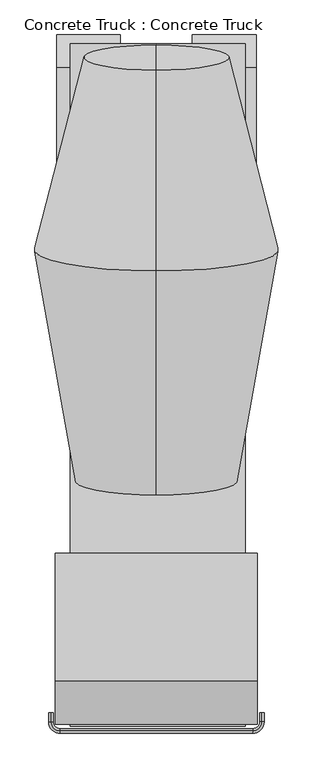
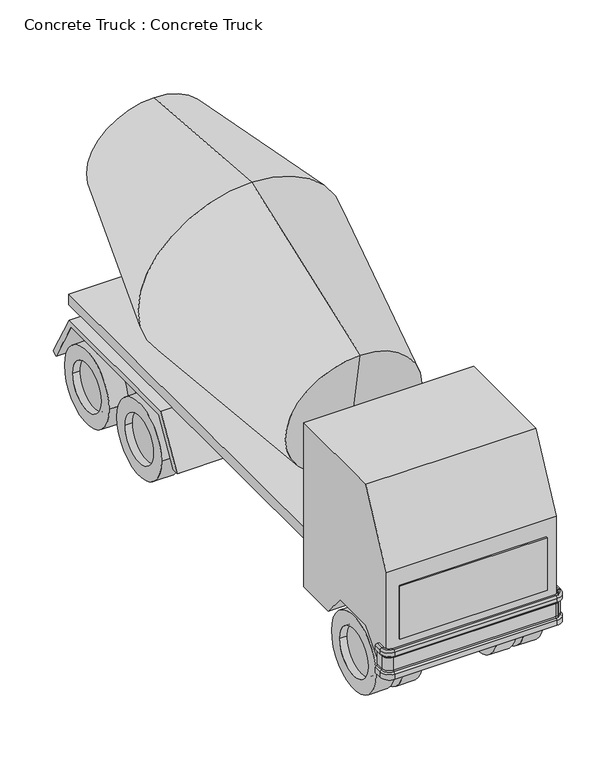
"""IFC4 building model written with IfcOpenShell, lengths in millimetres: geographic element geometry, Concrete Truck : Concrete Truck."""

from ifc_helpers import new_model, si_unit, point, frame, frame_2d, origin, place, context, project, spatial, polyline, circle_curve, ellipse_curve, trimmed, segment, composite_curve, outline, extrude, source, transform, mapped, element, save
from ifc_brep_helpers import plane_surface, cylinder_surface, revolved_surface, advanced_brep


def concrete_truck_concrete_truck_86626955(model_context):
    return source(origin(), model_context, "Body", "SolidModel", [
        extrude(outline(composite_curve([segment(trimmed(circle_curve(frame_2d((-3129.2190592, 514.3449875)), 330.2), [point((-2799.0190592, 514.3449875))], [point((-3459.4190592, 514.3449875))], False, "CARTESIAN"), True, "CONTINUOUS"), segment(trimmed(circle_curve(frame_2d((-3129.2190592, 514.3449875)), 330.2), [point((-3459.4190592, 514.3449875))], [point((-2799.0190592, 514.3449875))], False, "CARTESIAN"), True, "CONTINUOUS")], self_intersect=False)), frame((829.1634615, 0.0, 0.0), z_axis=(1.0, 0.0, 0.0), x_axis=(0.0, 1.0, 0.0)), (0.0, 0.0, 1.0), 172.4421875),
        extrude(outline(composite_curve([segment(trimmed(circle_curve(frame_2d((1874.5809408, 514.3449875)), 330.2), [point((2204.7809408, 514.3449875))], [point((1544.3809408, 514.3449875))], False, "CARTESIAN"), True, "CONTINUOUS"), segment(trimmed(circle_curve(frame_2d((1874.5809408, 514.3449875)), 330.2), [point((1544.3809408, 514.3449875))], [point((2204.7809408, 514.3449875))], False, "CARTESIAN"), True, "CONTINUOUS")], self_intersect=False)), frame((829.1634615, 0.0, 0.0), z_axis=(1.0, 0.0, 0.0), x_axis=(0.0, 1.0, 0.0)), (0.0, 0.0, 1.0), 172.4421875),
        extrude(outline(composite_curve([segment(trimmed(circle_curve(frame_2d((3091.9615385, 514.35)), 330.2), [point((3422.1615385, 514.35))], [point((2761.7615385, 514.35))], False, "CARTESIAN"), True, "CONTINUOUS"), segment(trimmed(circle_curve(frame_2d((3091.9615385, 514.35)), 330.2), [point((2761.7615385, 514.35))], [point((3422.1615385, 514.35))], False, "CARTESIAN"), True, "CONTINUOUS")], self_intersect=False)), frame((829.1634615, 0.0, 0.0), z_axis=(1.0, 0.0, 0.0), x_axis=(0.0, 1.0, 0.0)), (0.0, 0.0, 1.0), 172.4421875),
        extrude(outline(composite_curve([segment(trimmed(circle_curve(frame_2d((-3131.0384615, 514.35)), 330.2), [point((-2800.8384615, 514.35))], [point((-3461.2384615, 514.35))], False, "CARTESIAN"), True, "CONTINUOUS"), segment(trimmed(circle_curve(frame_2d((-3131.0384615, 514.35)), 330.2), [point((-3461.2384615, 514.35))], [point((-2800.8384615, 514.35))], False, "CARTESIAN"), True, "CONTINUOUS")], self_intersect=False)), frame((-1072.859976, 0.0, 0.0), z_axis=(1.0, 0.0, 0.0), x_axis=(0.0, 1.0, 0.0)), (0.0, 0.0, 1.0), 155.7734375),
        extrude(outline(composite_curve([segment(trimmed(circle_curve(frame_2d((1872.7615385, 514.35)), 330.2), [point((2202.9615385, 514.35))], [point((1542.5615385, 514.35))], False, "CARTESIAN"), True, "CONTINUOUS"), segment(trimmed(circle_curve(frame_2d((1872.7615385, 514.35)), 330.2), [point((1542.5615385, 514.35))], [point((2202.9615385, 514.35))], False, "CARTESIAN"), True, "CONTINUOUS")], self_intersect=False)), frame((-1072.859976, 0.0, 0.0), z_axis=(1.0, 0.0, 0.0), x_axis=(0.0, 1.0, 0.0)), (0.0, 0.0, 1.0), 155.7734375),
        extrude(outline(composite_curve([segment(trimmed(circle_curve(frame_2d((3091.9615385, 514.35)), 330.2), [point((3422.1615385, 514.35))], [point((2761.7615385, 514.35))], False, "CARTESIAN"), True, "CONTINUOUS"), segment(trimmed(circle_curve(frame_2d((3091.9615385, 514.35)), 330.2), [point((2761.7615385, 514.35))], [point((3422.1615385, 514.35))], False, "CARTESIAN"), True, "CONTINUOUS")], self_intersect=False)), frame((-1072.859976, 0.0, 0.0), z_axis=(1.0, 0.0, 0.0), x_axis=(0.0, 1.0, 0.0)), (0.0, 0.0, 1.0), 155.7734375),
        extrude(outline(composite_curve([segment(trimmed(circle_curve(frame_2d((3091.9615385, 514.35)), 520.7), [point((3612.6615385, 514.35))], [point((2571.2615385, 514.35))], False, "CARTESIAN"), True, "CONTINUOUS"), segment(trimmed(circle_curve(frame_2d((3091.9615385, 514.35)), 520.7), [point((2571.2615385, 514.35))], [point((3612.6615385, 514.35))], False, "CARTESIAN"), True, "CONTINUOUS")], self_intersect=False)), frame((-805.9615385, 0.0, 0.0), z_axis=(1.0, 0.0, 0.0), x_axis=(0.0, 1.0, 0.0)), (0.0, 0.0, 1.0), 254.0),
        extrude(outline(composite_curve([segment(trimmed(circle_curve(frame_2d((-3139.2915601, 511.4267776)), 520.7), [point((-2618.5915601, 511.4267776))], [point((-3659.9915601, 511.4267776))], False, "CARTESIAN"), True, "CONTINUOUS"), segment(trimmed(circle_curve(frame_2d((-3139.2915601, 511.4267776)), 520.7), [point((-3659.9915601, 511.4267776))], [point((-2618.5915601, 511.4267776))], False, "CARTESIAN"), True, "CONTINUOUS")], self_intersect=False)), frame((-805.9615385, 0.0, 0.0), z_axis=(1.0, 0.0, 0.0), x_axis=(0.0, 1.0, 0.0)), (0.0, 0.0, 1.0), 254.0),
        extrude(outline(composite_curve([segment(trimmed(circle_curve(frame_2d((1872.7615385, 514.35)), 520.7), [point((2393.4615385, 514.35))], [point((1352.0615385, 514.35))], False, "CARTESIAN"), True, "CONTINUOUS"), segment(trimmed(circle_curve(frame_2d((1872.7615385, 514.35)), 520.7), [point((1352.0615385, 514.35))], [point((2393.4615385, 514.35))], False, "CARTESIAN"), True, "CONTINUOUS")], self_intersect=False)), frame((-805.9615385, 0.0, 0.0), z_axis=(1.0, 0.0, 0.0), x_axis=(0.0, 1.0, 0.0)), (0.0, 0.0, 1.0), 254.0),
        extrude(outline(composite_curve([segment(trimmed(circle_curve(frame_2d((3091.9615385, 514.35)), 520.7), [point((3612.6615385, 514.35))], [point((2571.2615385, 514.35))], False, "CARTESIAN"), True, "CONTINUOUS"), segment(trimmed(circle_curve(frame_2d((3091.9615385, 514.35)), 520.7), [point((2571.2615385, 514.35))], [point((3612.6615385, 514.35))], False, "CARTESIAN"), True, "CONTINUOUS")], self_intersect=False)), frame((464.0384615, 0.0, 0.0), z_axis=(1.0, 0.0, 0.0), x_axis=(0.0, 1.0, 0.0)), (0.0, 0.0, 1.0), 254.0),
        extrude(outline(composite_curve([segment(trimmed(circle_curve(frame_2d((-3131.0384615, 514.35)), 520.7), [point((-2610.3384615, 514.35))], [point((-3651.7384615, 514.35))], False, "CARTESIAN"), True, "CONTINUOUS"), segment(trimmed(circle_curve(frame_2d((-3131.0384615, 514.35)), 520.7), [point((-3651.7384615, 514.35))], [point((-2610.3384615, 514.35))], False, "CARTESIAN"), True, "CONTINUOUS")], self_intersect=False)), frame((464.0384615, 0.0, 0.0), z_axis=(1.0, 0.0, 0.0), x_axis=(0.0, 1.0, 0.0)), (0.0, 0.0, 1.0), 254.0),
        extrude(outline(composite_curve([segment(trimmed(circle_curve(frame_2d((1872.7615385, 514.35)), 520.7), [point((2393.4615385, 514.35))], [point((1352.0615385, 514.35))], False, "CARTESIAN"), True, "CONTINUOUS"), segment(trimmed(circle_curve(frame_2d((1872.7615385, 514.35)), 520.7), [point((1352.0615385, 514.35))], [point((2393.4615385, 514.35))], False, "CARTESIAN"), True, "CONTINUOUS")], self_intersect=False)), frame((464.0384615, 0.0, 0.0), z_axis=(1.0, 0.0, 0.0), x_axis=(0.0, 1.0, 0.0)), (0.0, 0.0, 1.0), 254.0),
        extrude(outline(composite_curve([segment(trimmed(circle_curve(frame_2d((3091.9615385, 514.35)), 520.7), [point((3612.6615385, 514.35))], [point((2571.2615385, 514.35))], False, "CARTESIAN"), True, "CONTINUOUS"), segment(trimmed(circle_curve(frame_2d((3091.9615385, 514.35)), 520.7), [point((2571.2615385, 514.35))], [point((3612.6615385, 514.35))], False, "CARTESIAN"), True, "CONTINUOUS")], self_intersect=False), holes=[composite_curve([segment(trimmed(circle_curve(frame_2d((3091.9615385, 514.35)), 330.2), [point((3422.1615385, 514.35))], [point((2761.7615385, 514.35))], True, "CARTESIAN"), True, "CONTINUOUS"), segment(trimmed(circle_curve(frame_2d((3091.9615385, 514.35)), 330.2), [point((2761.7615385, 514.35))], [point((3422.1615385, 514.35))], True, "CARTESIAN"), True, "CONTINUOUS")], self_intersect=False)]), frame((-1171.0865385, 0.0, 0.0), z_axis=(1.0, 0.0, 0.0), x_axis=(0.0, 1.0, 0.0)), (0.0, 0.0, 1.0), 254.0),
        extrude(outline(composite_curve([segment(trimmed(circle_curve(frame_2d((-3131.0384615, 514.35)), 520.7), [point((-2610.3384615, 514.35))], [point((-3651.7384615, 514.35))], False, "CARTESIAN"), True, "CONTINUOUS"), segment(trimmed(circle_curve(frame_2d((-3131.0384615, 514.35)), 520.7), [point((-3651.7384615, 514.35))], [point((-2610.3384615, 514.35))], False, "CARTESIAN"), True, "CONTINUOUS")], self_intersect=False), holes=[composite_curve([segment(trimmed(circle_curve(frame_2d((-3131.0384615, 514.35)), 330.2), [point((-2800.8384615, 514.35))], [point((-3461.2384615, 514.35))], True, "CARTESIAN"), True, "CONTINUOUS"), segment(trimmed(circle_curve(frame_2d((-3131.0384615, 514.35)), 330.2), [point((-3461.2384615, 514.35))], [point((-2800.8384615, 514.35))], True, "CARTESIAN"), True, "CONTINUOUS")], self_intersect=False)]), frame((-1171.0865385, 0.0, 0.0), z_axis=(1.0, 0.0, 0.0), x_axis=(0.0, 1.0, 0.0)), (0.0, 0.0, 1.0), 254.0),
        extrude(outline(composite_curve([segment(trimmed(circle_curve(frame_2d((1872.7615385, 514.35)), 520.7), [point((2393.4615385, 514.35))], [point((1352.0615385, 514.35))], False, "CARTESIAN"), True, "CONTINUOUS"), segment(trimmed(circle_curve(frame_2d((1872.7615385, 514.35)), 520.7), [point((1352.0615385, 514.35))], [point((2393.4615385, 514.35))], False, "CARTESIAN"), True, "CONTINUOUS")], self_intersect=False), holes=[composite_curve([segment(trimmed(circle_curve(frame_2d((1872.7615385, 514.35)), 330.2), [point((2202.9615385, 514.35))], [point((1542.5615385, 514.35))], True, "CARTESIAN"), True, "CONTINUOUS"), segment(trimmed(circle_curve(frame_2d((1872.7615385, 514.35)), 330.2), [point((1542.5615385, 514.35))], [point((2202.9615385, 514.35))], True, "CARTESIAN"), True, "CONTINUOUS")], self_intersect=False)]), frame((-1171.0865385, 0.0, 0.0), z_axis=(1.0, 0.0, 0.0), x_axis=(0.0, 1.0, 0.0)), (0.0, 0.0, 1.0), 254.0),
        advanced_brep(
        [(-1212.3615385, -3791.4384615, 661.0144121), (-1263.1615385, -3791.4384615, 661.0144121), (-1263.1615385, -3791.4384615, 734.1328754), (-1243.6602579, -3791.4384615, 753.634156), (-1236.2207701, -3791.4384615, 771.5946682), (-1236.2207701, -3791.4384615, 953.7526192), (-1243.6602579, -3791.4384615, 971.7131315), (-1263.1615385, -3791.4384615, 991.2144121), (-1263.1615385, -3791.4384615, 1042.0144121), (-1237.7615385, -3791.4384615, 1067.4144121), (-1212.3615385, -3791.4384615, 1067.4144121), (-1212.3615385, -3893.0384615, 661.0144121), (-1263.1615385, -3893.0384615, 661.0144121), (-1263.1615385, -3893.0384615, 734.1328754), (-1243.6602579, -3893.0384615, 753.634156), (-1236.2207701, -3893.0384615, 771.5946682), (-1236.2207701, -3893.0384615, 953.7526192), (-1243.6602579, -3893.0384615, 971.7131315), (-1263.1615385, -3893.0384615, 991.2144121), (-1263.1615385, -3893.0384615, 1042.0144121), (-1237.7615385, -3893.0384615, 1067.4144121), (-1212.3615385, -3893.0384615, 1067.4144121), (-1136.1615385, -4020.0384615, 661.0144121), (-1136.1615385, -3969.2384615, 661.0144121), (-1136.1615385, -4020.0384615, 734.1328754), (-1136.1615385, -4000.5371809, 753.634156), (-1136.1615385, -3993.0976932, 771.5946682), (-1136.1615385, -3993.0976932, 953.7526192), (-1136.1615385, -4000.5371809, 971.7131315), (-1136.1615385, -4020.0384615, 991.2144121), (-1136.1615385, -4020.0384615, 1042.0144121), (-1136.1615385, -3994.6384615, 1067.4144121), (-1136.1615385, -3969.2384615, 1067.4144121), (1048.2384615, -3969.2384615, 661.0144121), (1048.2384615, -4020.0384615, 661.0144121), (1048.2384615, -4020.0384615, 734.1328754), (1048.2384615, -4000.5371809, 753.634156), (1048.2384615, -3993.0976932, 771.5946682), (1048.2384615, -3993.0976932, 953.7526192), (1048.2384615, -4000.5371809, 971.7131315), (1048.2384615, -4020.0384615, 991.2144121), (1048.2384615, -4020.0384615, 1042.0144121), (1048.2384615, -3994.6384615, 1067.4144121), (1048.2384615, -3969.2384615, 1067.4144121), (1175.2384615, -3893.0384615, 661.0144121), (1124.4384615, -3893.0384615, 661.0144121), (1175.2384615, -3893.0384615, 734.1328754), (1155.7371809, -3893.0384615, 753.634156), (1148.2976932, -3893.0384615, 771.5946682), (1148.2976932, -3893.0384615, 953.7526192), (1155.7371809, -3893.0384615, 971.7131315), (1175.2384615, -3893.0384615, 991.2144121), (1175.2384615, -3893.0384615, 1042.0144121), (1149.8384615, -3893.0384615, 1067.4144121), (1124.4384615, -3893.0384615, 1067.4144121), (1124.4384615, -3791.4384615, 661.0144121), (1124.4384615, -3791.4384615, 1067.4144121), (1149.8384615, -3791.4384615, 1067.4144121), (1175.2384615, -3791.4384615, 1042.0144121), (1175.2384615, -3791.4384615, 991.2144121), (1155.7371809, -3791.4384615, 971.7131315), (1148.2976932, -3791.4384615, 953.7526192), (1148.2976932, -3791.4384615, 771.5946682), (1155.7371809, -3791.4384615, 753.634156), (1175.2384615, -3791.4384615, 734.1328754), (1175.2384615, -3791.4384615, 661.0144121)],
        [
            (0, 1),
            (1, 2),
            (2, 3),
            (3, 4, circle_curve(frame((-1261.6207701, -3791.4384615, 771.5946682), z_axis=(0.0, -1.0, 0.0), x_axis=(1.0, 0.0, 0.0)), 25.4)),
            (4, 5),
            (5, 6, circle_curve(frame((-1261.6207701, -3791.4384615, 953.7526192), z_axis=(0.0, -1.0, 0.0), x_axis=(1.0, 0.0, 0.0)), 25.4)),
            (6, 7),
            (7, 8),
            (8, 9, circle_curve(frame((-1237.7615385, -3791.4384615, 1042.0144121), z_axis=(0.0, 1.0, 0.0), x_axis=(1.0, 0.0, 0.0)), 25.4)),
            (9, 10),
            (10, 0),
            (0, 11),
            (11, 12),
            (12, 1),
            (12, 13),
            (13, 2),
            (13, 14),
            (14, 3),
            (14, 15, circle_curve(frame((-1261.6207701, -3893.0384615, 771.5946682), z_axis=(0.0, -1.0, 0.0), x_axis=(1.0, 0.0, 0.0)), 25.4)),
            (15, 4),
            (15, 16),
            (16, 5),
            (16, 17, circle_curve(frame((-1261.6207701, -3893.0384615, 953.7526192), z_axis=(0.0, -1.0, 0.0), x_axis=(1.0, 0.0, 0.0)), 25.4)),
            (17, 6),
            (17, 18),
            (18, 7),
            (18, 19),
            (19, 8),
            (19, 20, circle_curve(frame((-1237.7615385, -3893.0384615, 1042.0144121), z_axis=(0.0, 1.0, 0.0), x_axis=(1.0, 0.0, 0.0)), 25.4)),
            (20, 9),
            (20, 21),
            (21, 10),
            (21, 11),
            (22, 12, circle_curve(frame((-1136.1615385, -3893.0384615, 661.0144121), z_axis=(0.0, 0.0, -1.0), x_axis=(-1.0, 0.0, 0.0)), 127.0)),
            (11, 23, circle_curve(frame((-1136.1615385, -3893.0384615, 661.0144121), z_axis=(0.0, 0.0, 1.0), x_axis=(-1.0, 0.0, 0.0)), 76.2)),
            (23, 22),
            (24, 13, circle_curve(frame((-1136.1615385, -3893.0384615, 734.1328754), z_axis=(0.0, 0.0, -1.0), x_axis=(-1.0, 0.0, 0.0)), 127.0)),
            (22, 24),
            (25, 14, circle_curve(frame((-1136.1615385, -3893.0384615, 753.634156), z_axis=(0.0, 0.0, -1.0), x_axis=(-1.0, 0.0, 0.0)), 107.4987194)),
            (24, 25),
            (26, 15, circle_curve(frame((-1136.1615385, -3893.0384615, 771.5946682), z_axis=(0.0, 0.0, -1.0), x_axis=(-1.0, 0.0, 0.0)), 100.0592316)),
            (25, 26, circle_curve(frame((-1136.1615385, -4018.4976932, 771.5946682), z_axis=(1.0, 0.0, 0.0), x_axis=(0.0, 1.0, 0.0)), 25.4)),
            (27, 16, circle_curve(frame((-1136.1615385, -3893.0384615, 953.7526192), z_axis=(0.0, 0.0, -1.0), x_axis=(-1.0, 0.0, 0.0)), 100.0592316)),
            (26, 27),
            (28, 17, circle_curve(frame((-1136.1615385, -3893.0384615, 971.7131315), z_axis=(0.0, 0.0, -1.0), x_axis=(-1.0, 0.0, 0.0)), 107.4987194)),
            (27, 28, circle_curve(frame((-1136.1615385, -4018.4976932, 953.7526192), z_axis=(1.0, 0.0, 0.0), x_axis=(0.0, 1.0, 0.0)), 25.4)),
            (29, 18, circle_curve(frame((-1136.1615385, -3893.0384615, 991.2144121), z_axis=(0.0, 0.0, -1.0), x_axis=(-1.0, 0.0, 0.0)), 127.0)),
            (28, 29),
            (30, 19, circle_curve(frame((-1136.1615385, -3893.0384615, 1042.0144121), z_axis=(0.0, 0.0, -1.0), x_axis=(-1.0, 0.0, 0.0)), 127.0)),
            (29, 30),
            (31, 20, circle_curve(frame((-1136.1615385, -3893.0384615, 1067.4144121), z_axis=(0.0, 0.0, -1.0), x_axis=(-1.0, 0.0, 0.0)), 101.6)),
            (30, 31, circle_curve(frame((-1136.1615385, -3994.6384615, 1042.0144121), z_axis=(-1.0, 0.0, 0.0), x_axis=(0.0, 1.0, 0.0)), 25.4)),
            (32, 21, circle_curve(frame((-1136.1615385, -3893.0384615, 1067.4144121), z_axis=(0.0, 0.0, -1.0), x_axis=(-1.0, 0.0, 0.0)), 76.2)),
            (31, 32),
            (32, 23),
            (23, 33),
            (33, 34),
            (34, 22),
            (34, 35),
            (35, 24),
            (35, 36),
            (36, 25),
            (36, 37, circle_curve(frame((1048.2384615, -4018.4976932, 771.5946682), z_axis=(1.0, 0.0, 0.0), x_axis=(0.0, 1.0, 0.0)), 25.4)),
            (37, 26),
            (37, 38),
            (38, 27),
            (38, 39, circle_curve(frame((1048.2384615, -4018.4976932, 953.7526192), z_axis=(1.0, 0.0, 0.0), x_axis=(0.0, 1.0, 0.0)), 25.4)),
            (39, 28),
            (39, 40),
            (40, 29),
            (40, 41),
            (41, 30),
            (41, 42, circle_curve(frame((1048.2384615, -3994.6384615, 1042.0144121), z_axis=(-1.0, 0.0, 0.0), x_axis=(0.0, 1.0, 0.0)), 25.4)),
            (42, 31),
            (42, 43),
            (43, 32),
            (43, 33),
            (44, 34, circle_curve(frame((1048.2384615, -3893.0384615, 661.0144121), z_axis=(0.0, 0.0, -1.0), x_axis=(0.0, -1.0, 0.0)), 127.0)),
            (33, 45, circle_curve(frame((1048.2384615, -3893.0384615, 661.0144121), z_axis=(0.0, 0.0, 1.0), x_axis=(0.0, -1.0, 0.0)), 76.2)),
            (45, 44),
            (46, 35, circle_curve(frame((1048.2384615, -3893.0384615, 734.1328754), z_axis=(0.0, 0.0, -1.0), x_axis=(0.0, -1.0, 0.0)), 127.0)),
            (44, 46),
            (47, 36, circle_curve(frame((1048.2384615, -3893.0384615, 753.634156), z_axis=(0.0, 0.0, -1.0), x_axis=(0.0, -1.0, 0.0)), 107.4987194)),
            (46, 47),
            (48, 37, circle_curve(frame((1048.2384615, -3893.0384615, 771.5946682), z_axis=(0.0, 0.0, -1.0), x_axis=(0.0, -1.0, 0.0)), 100.0592316)),
            (47, 48, circle_curve(frame((1173.6976932, -3893.0384615, 771.5946682), z_axis=(0.0, 1.0, 0.0), x_axis=(-1.0, 0.0, 0.0)), 25.4)),
            (49, 38, circle_curve(frame((1048.2384615, -3893.0384615, 953.7526192), z_axis=(0.0, 0.0, -1.0), x_axis=(0.0, -1.0, 0.0)), 100.0592316)),
            (48, 49),
            (50, 39, circle_curve(frame((1048.2384615, -3893.0384615, 971.7131315), z_axis=(0.0, 0.0, -1.0), x_axis=(0.0, -1.0, 0.0)), 107.4987194)),
            (49, 50, circle_curve(frame((1173.6976932, -3893.0384615, 953.7526192), z_axis=(0.0, 1.0, 0.0), x_axis=(-1.0, 0.0, 0.0)), 25.4)),
            (51, 40, circle_curve(frame((1048.2384615, -3893.0384615, 991.2144121), z_axis=(0.0, 0.0, -1.0), x_axis=(0.0, -1.0, 0.0)), 127.0)),
            (50, 51),
            (52, 41, circle_curve(frame((1048.2384615, -3893.0384615, 1042.0144121), z_axis=(0.0, 0.0, -1.0), x_axis=(0.0, -1.0, 0.0)), 127.0)),
            (51, 52),
            (53, 42, circle_curve(frame((1048.2384615, -3893.0384615, 1067.4144121), z_axis=(0.0, 0.0, -1.0), x_axis=(0.0, -1.0, 0.0)), 101.6)),
            (52, 53, circle_curve(frame((1149.8384615, -3893.0384615, 1042.0144121), z_axis=(0.0, -1.0, 0.0), x_axis=(-1.0, 0.0, 0.0)), 25.4)),
            (54, 43, circle_curve(frame((1048.2384615, -3893.0384615, 1067.4144121), z_axis=(0.0, 0.0, -1.0), x_axis=(0.0, -1.0, 0.0)), 76.2)),
            (53, 54),
            (54, 45),
            (55, 56),
            (56, 57),
            (57, 58, circle_curve(frame((1149.8384615, -3791.4384615, 1042.0144121), z_axis=(0.0, 1.0, 0.0), x_axis=(-1.0, 0.0, 0.0)), 25.4)),
            (58, 59),
            (59, 60),
            (60, 61, circle_curve(frame((1173.6976932, -3791.4384615, 953.7526192), z_axis=(0.0, -1.0, 0.0), x_axis=(-1.0, 0.0, 0.0)), 25.4)),
            (61, 62),
            (62, 63, circle_curve(frame((1173.6976932, -3791.4384615, 771.5946682), z_axis=(0.0, -1.0, 0.0), x_axis=(-1.0, 0.0, 0.0)), 25.4)),
            (63, 64),
            (64, 65),
            (65, 55),
            (45, 55),
            (65, 44),
            (64, 46),
            (63, 47),
            (62, 48),
            (61, 49),
            (60, 50),
            (59, 51),
            (58, 52),
            (57, 53),
            (56, 54),
        ],
        [
            plane_surface(frame((-2331.7840944, -3791.4384615, 0.0), z_axis=(0.0, 1.0, 0.0), x_axis=(0.0, 0.0, -1.0))),
            plane_surface(frame((-1212.3615385, -3791.4384615, 661.0144121), z_axis=(0.0, 0.0, -1.0), x_axis=(0.0, -1.0, 0.0))),
            plane_surface(frame((-1263.1615385, -3791.4384615, 661.0144121), z_axis=(-1.0, 0.0, 0.0), x_axis=(0.0, -1.0, 0.0))),
            plane_surface(frame((-1263.1615385, -3791.4384615, 734.1328754), z_axis=(-0.7071067811866113, 0.0, 0.7071067811864837), x_axis=(0.0, -1.0, 0.0))),
            revolved_surface(polyline([(-1236.2207701, -3893.0384615, 771.5946682), (-1236.2207701, -3791.4384615, 771.5946682)]), (-1261.6207701, -3791.4384615, 771.5946682), (0.0, -1.0, 0.0)),
            plane_surface(frame((-1236.2207701, -3791.4384615, 771.5946682), z_axis=(-1.0, 0.0, 0.0), x_axis=(0.0, -1.0, 0.0))),
            revolved_surface(polyline([(-1236.2207701, -3893.0384615, 953.7526192), (-1236.2207701, -3791.4384615, 953.7526192)]), (-1261.6207701, -3791.4384615, 953.7526192), (0.0, -1.0, 0.0)),
            plane_surface(frame((-1243.6602579, -3791.4384615, 971.7131315), z_axis=(-0.7071067811866555, 0.0, -0.7071067811864395), x_axis=(0.0, -1.0, 0.0))),
            plane_surface(frame((-1263.1615385, -3791.4384615, 991.2144121), z_axis=(-1.0, 0.0, 0.0), x_axis=(0.0, -1.0, 0.0))),
            cylinder_surface(frame((-1237.7615385, -3791.4384615, 1042.0144121), z_axis=(0.0, 1.0, 0.0), x_axis=(1.0, 0.0, 0.0)), 25.4),
            plane_surface(frame((-1237.7615385, -3791.4384615, 1067.4144121), z_axis=(0.0, 0.0, 1.0), x_axis=(0.0, -1.0, 0.0))),
            plane_surface(frame((-1212.3615385, -3791.4384615, 1067.4144121), z_axis=(1.0, 0.0, 0.0), x_axis=(0.0, -1.0, 0.0))),
            plane_surface(frame((-1136.1615385, -3893.0384615, 661.0144121), z_axis=(0.0, 0.0, -1.0), x_axis=(-1.0, 0.0, 0.0))),
            cylinder_surface(frame((-1136.1615385, -3893.0384615, 0.0), z_axis=(0.0, 0.0, 1.0), x_axis=(-1.0, 0.0, 0.0)), 127.0),
            revolved_surface(polyline([(-1263.1615385, -3893.0384615, 734.1328754), (-1243.6602579, -3893.0384615, 753.634156)]), (-1136.1615385, -3893.0384615, 0.0), (0.0, 0.0, 1.0)),
            revolved_surface(trimmed(ellipse_curve(frame((-1261.6207701, -3893.0384615, 771.5946682), z_axis=(0.0, -1.0, 0.0), x_axis=(1.0, 0.0, 0.0)), 25.4, 25.4), [point((-1243.6602579, -3893.0384615, 753.634156))], [point((-1236.2207701, -3893.0384615, 771.5946682))], True, "CARTESIAN"), (-1136.1615385, -3893.0384615, 0.0), (0.0, 0.0, 1.0)),
            cylinder_surface(frame((-1136.1615385, -3893.0384615, 0.0), z_axis=(0.0, 0.0, 1.0), x_axis=(-1.0, 0.0, 0.0)), 100.0592316),
            revolved_surface(trimmed(ellipse_curve(frame((-1261.6207701, -3893.0384615, 953.7526192), z_axis=(0.0, -1.0, 0.0), x_axis=(1.0, 0.0, 0.0)), 25.4, 25.4), [point((-1236.2207701, -3893.0384615, 953.7526192))], [point((-1243.6602579, -3893.0384615, 971.7131315))], True, "CARTESIAN"), (-1136.1615385, -3893.0384615, 0.0), (0.0, 0.0, 1.0)),
            revolved_surface(polyline([(-1243.6602579, -3893.0384615, 971.7131315), (-1263.1615385, -3893.0384615, 991.2144121)]), (-1136.1615385, -3893.0384615, 0.0), (0.0, 0.0, 1.0)),
            revolved_surface(trimmed(ellipse_curve(frame((-1237.7615385, -3893.0384615, 1042.0144121), z_axis=(0.0, 1.0, 0.0), x_axis=(1.0, 0.0, 0.0)), 25.4, 25.4), [point((-1263.1615385, -3893.0384615, 1042.0144121))], [point((-1237.7615385, -3893.0384615, 1067.4144121))], True, "CARTESIAN"), (-1136.1615385, -3893.0384615, 0.0), (0.0, 0.0, 1.0)),
            plane_surface(frame((-1136.1615385, -3893.0384615, 1067.4144121), z_axis=(0.0, 0.0, 1.0), x_axis=(-1.0, 0.0, 0.0))),
            revolved_surface(polyline([(-1212.3615385, -3893.0384615, 1067.4144121), (-1212.3615385, -3893.0384615, 661.0144121)]), (-1136.1615385, -3893.0384615, 0.0), (0.0, 0.0, 1.0)),
            plane_surface(frame((-1136.1615385, -3969.2384615, 661.0144121), z_axis=(0.0, 0.0, -1.0), x_axis=(1.0, 0.0, 0.0))),
            plane_surface(frame((-1136.1615385, -4020.0384615, 661.0144121), z_axis=(0.0, -1.0, 0.0), x_axis=(1.0, 0.0, 0.0))),
            plane_surface(frame((-1136.1615385, -4020.0384615, 734.1328754), z_axis=(0.0, -0.7071067811866113, 0.7071067811864837), x_axis=(1.0, 0.0, 0.0))),
            revolved_surface(polyline([(1048.2384615, -3993.0976932, 771.5946682), (-1136.1615385, -3993.0976932, 771.5946682)]), (-1136.1615385, -4018.4976932, 771.5946682), (1.0, 0.0, 0.0)),
            plane_surface(frame((-1136.1615385, -3993.0976932, 771.5946682), z_axis=(0.0, -1.0, 0.0), x_axis=(1.0, 0.0, 0.0))),
            revolved_surface(polyline([(1048.2384615, -3993.0976932, 953.7526192), (-1136.1615385, -3993.0976932, 953.7526192)]), (-1136.1615385, -4018.4976932, 953.7526192), (1.0, 0.0, 0.0)),
            plane_surface(frame((-1136.1615385, -4000.5371809, 971.7131315), z_axis=(0.0, -0.7071067811866555, -0.7071067811864395), x_axis=(1.0, 0.0, 0.0))),
            plane_surface(frame((-1136.1615385, -4020.0384615, 991.2144121), z_axis=(0.0, -1.0, 0.0), x_axis=(1.0, 0.0, 0.0))),
            cylinder_surface(frame((-1136.1615385, -3994.6384615, 1042.0144121), z_axis=(-1.0, 0.0, 0.0), x_axis=(0.0, 1.0, 0.0)), 25.4),
            plane_surface(frame((-1136.1615385, -3994.6384615, 1067.4144121), z_axis=(0.0, 0.0, 1.0), x_axis=(1.0, 0.0, 0.0))),
            plane_surface(frame((-1136.1615385, -3969.2384615, 1067.4144121), z_axis=(0.0, 1.0, 0.0), x_axis=(1.0, 0.0, 0.0))),
            plane_surface(frame((1048.2384615, -3893.0384615, 661.0144121), z_axis=(0.0, 0.0, -1.0), x_axis=(0.0, -1.0, 0.0))),
            cylinder_surface(frame((1048.2384615, -3893.0384615, 0.0), z_axis=(0.0, 0.0, 1.0), x_axis=(0.0, -1.0, 0.0)), 127.0),
            revolved_surface(polyline([(1048.2384615, -4020.0384615, 734.1328754), (1048.2384615, -4000.5371809, 753.634156)]), (1048.2384615, -3893.0384615, 0.0), (0.0, 0.0, 1.0)),
            revolved_surface(trimmed(ellipse_curve(frame((1048.2384615, -4018.4976932, 771.5946682), z_axis=(1.0, 0.0, 0.0), x_axis=(0.0, 1.0, 0.0)), 25.4, 25.4), [point((1048.2384615, -4000.5371809, 753.634156))], [point((1048.2384615, -3993.0976932, 771.5946682))], True, "CARTESIAN"), (1048.2384615, -3893.0384615, 0.0), (0.0, 0.0, 1.0)),
            cylinder_surface(frame((1048.2384615, -3893.0384615, 0.0), z_axis=(0.0, 0.0, 1.0), x_axis=(0.0, -1.0, 0.0)), 100.0592316),
            revolved_surface(trimmed(ellipse_curve(frame((1048.2384615, -4018.4976932, 953.7526192), z_axis=(1.0, 0.0, 0.0), x_axis=(0.0, 1.0, 0.0)), 25.4, 25.4), [point((1048.2384615, -3993.0976932, 953.7526192))], [point((1048.2384615, -4000.5371809, 971.7131315))], True, "CARTESIAN"), (1048.2384615, -3893.0384615, 0.0), (0.0, 0.0, 1.0)),
            revolved_surface(polyline([(1048.2384615, -4000.5371809, 971.7131315), (1048.2384615, -4020.0384615, 991.2144121)]), (1048.2384615, -3893.0384615, 0.0), (0.0, 0.0, 1.0)),
            revolved_surface(trimmed(ellipse_curve(frame((1048.2384615, -3994.6384615, 1042.0144121), z_axis=(-1.0, 0.0, 0.0), x_axis=(0.0, 1.0, 0.0)), 25.4, 25.4), [point((1048.2384615, -4020.0384615, 1042.0144121))], [point((1048.2384615, -3994.6384615, 1067.4144121))], True, "CARTESIAN"), (1048.2384615, -3893.0384615, 0.0), (0.0, 0.0, 1.0)),
            plane_surface(frame((1048.2384615, -3893.0384615, 1067.4144121), z_axis=(0.0, 0.0, 1.0), x_axis=(0.0, -1.0, 0.0))),
            revolved_surface(polyline([(1048.2384615, -3969.2384614999996, 1067.4144121), (1048.2384615, -3969.2384614999996, 661.0144121)]), (1048.2384615, -3893.0384615, 0.0), (0.0, 0.0, 1.0)),
            plane_surface(frame((106.6159056, -3791.4384615, 0.0), z_axis=(0.0, 1.0, 0.0), x_axis=(0.0, 0.0, 1.0))),
            plane_surface(frame((1124.4384615, -3893.0384615, 661.0144121), z_axis=(0.0, 0.0, -1.0), x_axis=(0.0, 1.0, 0.0))),
            plane_surface(frame((1175.2384615, -3893.0384615, 661.0144121), z_axis=(1.0, 0.0, 0.0), x_axis=(0.0, 1.0, 0.0))),
            plane_surface(frame((1175.2384615, -3893.0384615, 734.1328754), z_axis=(0.7071067811866113, 0.0, 0.7071067811864837), x_axis=(0.0, 1.0, 0.0))),
            revolved_surface(polyline([(1148.2976932, -3791.4384615, 771.5946682), (1148.2976932, -3893.0384615, 771.5946682)]), (1173.6976932, -3893.0384615, 771.5946682), (0.0, 1.0, 0.0)),
            plane_surface(frame((1148.2976932, -3893.0384615, 771.5946682), z_axis=(1.0, 0.0, 0.0), x_axis=(0.0, 1.0, 0.0))),
            revolved_surface(polyline([(1148.2976932, -3791.4384615, 953.7526192), (1148.2976932, -3893.0384615, 953.7526192)]), (1173.6976932, -3893.0384615, 953.7526192), (0.0, 1.0, 0.0)),
            plane_surface(frame((1155.7371809, -3893.0384615, 971.7131315), z_axis=(0.7071067811866555, 0.0, -0.7071067811864395), x_axis=(0.0, 1.0, 0.0))),
            plane_surface(frame((1175.2384615, -3893.0384615, 991.2144121), z_axis=(1.0, 0.0, 0.0), x_axis=(0.0, 1.0, 0.0))),
            cylinder_surface(frame((1149.8384615, -3893.0384615, 1042.0144121), z_axis=(0.0, -1.0, 0.0), x_axis=(-1.0, 0.0, 0.0)), 25.4),
            plane_surface(frame((1149.8384615, -3893.0384615, 1067.4144121), z_axis=(0.0, 0.0, 1.0), x_axis=(0.0, 1.0, 0.0))),
            plane_surface(frame((1124.4384615, -3893.0384615, 1067.4144121), z_axis=(-1.0, 0.0, 0.0), x_axis=(0.0, 1.0, 0.0))),
        ],
        [
            (0, [[1, 2, 3, 4, 5, 6, 7, 8, 9, 10, 11]]),
            (1, [[-1, 12, 13, 14]]),
            (2, [[-2, -14, 15, 16]]),
            (3, [[-3, -16, 17, 18]]),
            (4, [[-4, -18, 19, 20]]),
            (5, [[-5, -20, 21, 22]]),
            (6, [[-6, -22, 23, 24]]),
            (7, [[-7, -24, 25, 26]]),
            (8, [[-8, -26, 27, 28]]),
            (9, [[-9, -28, 29, 30]]),
            (10, [[-10, -30, 31, 32]]),
            (11, [[-11, -32, 33, -12]]),
            (12, [[34, -13, 35, 36]]),
            (13, [[37, -15, -34, 38]]),
            (14, [[39, -17, -37, 40]]),
            (15, [[41, -19, -39, 42]]),
            (16, [[43, -21, -41, 44]]),
            (17, [[45, -23, -43, 46]]),
            (18, [[47, -25, -45, 48]]),
            (13, [[49, -27, -47, 50]]),
            (19, [[51, -29, -49, 52]]),
            (20, [[53, -31, -51, 54]]),
            (21, [[-35, -33, -53, 55]]),
            (22, [[-36, 56, 57, 58]]),
            (23, [[-38, -58, 59, 60]]),
            (24, [[-40, -60, 61, 62]]),
            (25, [[-42, -62, 63, 64]]),
            (26, [[-44, -64, 65, 66]]),
            (27, [[-46, -66, 67, 68]]),
            (28, [[-48, -68, 69, 70]]),
            (29, [[-50, -70, 71, 72]]),
            (30, [[-52, -72, 73, 74]]),
            (31, [[-54, -74, 75, 76]]),
            (32, [[-55, -76, 77, -56]]),
            (33, [[78, -57, 79, 80]]),
            (34, [[81, -59, -78, 82]]),
            (35, [[83, -61, -81, 84]]),
            (36, [[85, -63, -83, 86]]),
            (37, [[87, -65, -85, 88]]),
            (38, [[89, -67, -87, 90]]),
            (39, [[91, -69, -89, 92]]),
            (34, [[93, -71, -91, 94]]),
            (40, [[95, -73, -93, 96]]),
            (41, [[97, -75, -95, 98]]),
            (42, [[-79, -77, -97, 99]]),
            (43, [[100, 101, 102, 103, 104, 105, 106, 107, 108, 109, 110]]),
            (44, [[-80, 111, -110, 112]]),
            (45, [[-82, -112, -109, 113]]),
            (46, [[-84, -113, -108, 114]]),
            (47, [[-86, -114, -107, 115]]),
            (48, [[-88, -115, -106, 116]]),
            (49, [[-90, -116, -105, 117]]),
            (50, [[-92, -117, -104, 118]]),
            (51, [[-94, -118, -103, 119]]),
            (52, [[-96, -119, -102, 120]]),
            (53, [[-98, -120, -101, 121]]),
            (54, [[-99, -121, -100, -111]]),
        ],
    ),
        extrude(outline(composite_curve([segment(trimmed(circle_curve(frame_2d((3091.9615385, 514.35)), 520.7), [point((3612.6615385, 514.35))], [point((2571.2615385, 514.35))], False, "CARTESIAN"), True, "CONTINUOUS"), segment(trimmed(circle_curve(frame_2d((3091.9615385, 514.35)), 520.7), [point((2571.2615385, 514.35))], [point((3612.6615385, 514.35))], False, "CARTESIAN"), True, "CONTINUOUS")], self_intersect=False), holes=[composite_curve([segment(trimmed(circle_curve(frame_2d((3091.9615385, 514.35)), 330.2), [point((3422.1615385, 514.35))], [point((2761.7615385, 514.35))], True, "CARTESIAN"), True, "CONTINUOUS"), segment(trimmed(circle_curve(frame_2d((3091.9615385, 514.35)), 330.2), [point((2761.7615385, 514.35))], [point((3422.1615385, 514.35))], True, "CARTESIAN"), True, "CONTINUOUS")], self_intersect=False)]), frame((829.1634615, 0.0, 0.0), z_axis=(1.0, 0.0, 0.0), x_axis=(0.0, 1.0, 0.0)), (0.0, 0.0, 1.0), 254.0),
        extrude(outline(composite_curve([segment(trimmed(circle_curve(frame_2d((-3131.0384615, 514.35)), 520.7), [point((-2610.3384615, 514.35))], [point((-3651.7384615, 514.35))], False, "CARTESIAN"), True, "CONTINUOUS"), segment(trimmed(circle_curve(frame_2d((-3131.0384615, 514.35)), 520.7), [point((-3651.7384615, 514.35))], [point((-2610.3384615, 514.35))], False, "CARTESIAN"), True, "CONTINUOUS")], self_intersect=False), holes=[composite_curve([segment(trimmed(circle_curve(frame_2d((-3131.0384615, 514.35)), 330.2), [point((-2800.8384615, 514.35))], [point((-3461.2384615, 514.35))], True, "CARTESIAN"), True, "CONTINUOUS"), segment(trimmed(circle_curve(frame_2d((-3131.0384615, 514.35)), 330.2), [point((-3461.2384615, 514.35))], [point((-2800.8384615, 514.35))], True, "CARTESIAN"), True, "CONTINUOUS")], self_intersect=False)]), frame((829.1634615, 0.0, 0.0), z_axis=(1.0, 0.0, 0.0), x_axis=(0.0, 1.0, 0.0)), (0.0, 0.0, 1.0), 254.0),
        extrude(outline(composite_curve([segment(trimmed(circle_curve(frame_2d((1872.7615385, 514.35)), 520.7), [point((2393.4615385, 514.35))], [point((1352.0615385, 514.35))], False, "CARTESIAN"), True, "CONTINUOUS"), segment(trimmed(circle_curve(frame_2d((1872.7615385, 514.35)), 520.7), [point((1352.0615385, 514.35))], [point((2393.4615385, 514.35))], False, "CARTESIAN"), True, "CONTINUOUS")], self_intersect=False), holes=[composite_curve([segment(trimmed(circle_curve(frame_2d((1872.7615385, 514.35)), 330.2), [point((2202.9615385, 514.35))], [point((1542.5615385, 514.35))], True, "CARTESIAN"), True, "CONTINUOUS"), segment(trimmed(circle_curve(frame_2d((1872.7615385, 514.35)), 330.2), [point((1542.5615385, 514.35))], [point((2202.9615385, 514.35))], True, "CARTESIAN"), True, "CONTINUOUS")], self_intersect=False)]), frame((829.1634615, 0.0, 0.0), z_axis=(1.0, 0.0, 0.0), x_axis=(0.0, 1.0, 0.0)), (0.0, 0.0, 1.0), 254.0),
        extrude(outline(polyline([(362.4384615, 3777.7615385), (362.4384615, -1683.2384615), (725.7603556, -1683.2384615), (725.7603556, -3004.0384615), (-798.2396444, -3004.0384615), (-798.2396444, -1683.2384615), (-450.3615385, -1683.2384615), (-450.3615385, 3777.7615385), (362.4384615, 3777.7615385)])), frame((0.0, 0.0, 711.2), z_axis=(0.0, 0.0, 1.0), x_axis=(1.0, 0.0, 0.0)), (0.0, 0.0, 1.0), 508.0),
        advanced_brep(
        [(-43.9615385, -1168.0113462, 2355.2104547), (-43.9615385, -1009.570534, 1454.7367752), (-43.9615385, -1326.4521585, 3255.6841343), (-43.9615385, 1686.1636133, 1454.7367752), (-43.9615385, 1207.3779879, 4175.8403069), (-43.9615385, 3762.828493, 2387.7409698), (-43.9615385, 3477.789427, 4007.7161067), (-43.9615385, 3620.30896, 3197.7285383)],
        [
            (0, 1),
            (1, 2, circle_curve(frame((-43.9615385, -1168.0113462, 2355.2104547), z_axis=(0.0, -0.9848707186111331, -0.17329070264267052), x_axis=(0.0, 0.17329070264267052, -0.9848707186111331)), 914.3064795)),
            (2, 0),
            (2, 1, circle_curve(frame((-43.9615385, -1168.0113462, 2355.2104547), z_axis=(0.0, -0.9848707186111331, -0.17329070264267052), x_axis=(0.0, 0.17329070264267052, -0.9848707186111331)), 914.3064795)),
            (1, 3),
            (3, 4, circle_curve(frame((-43.9615385, 1446.7708006, 2815.2885411), z_axis=(0.0, -0.9848707186111331, -0.17329070264267052), x_axis=(0.0, 0.17329070264267052, -0.9848707186111331)), 1381.452144)),
            (4, 2),
            (4, 3, circle_curve(frame((-43.9615385, 1446.7708006, 2815.2885411), z_axis=(0.0, -0.9848707186111331, -0.17329070264267052), x_axis=(0.0, 0.17329070264267052, -0.9848707186111331)), 1381.452144)),
            (3, 5),
            (5, 6, circle_curve(frame((-43.9615385, 3620.30896, 3197.7285383), z_axis=(0.0, -0.9848707186111331, -0.17329070264267052), x_axis=(0.0, 0.17329070264267052, -0.9848707186111331)), 822.4303486)),
            (6, 4),
            (5, 7),
            (7, 6),
            (5, 6, circle_curve(frame((-43.9615385, 3620.30896, 3197.7285383), z_axis=(0.0, 0.9848707186111331, 0.17329070264267052), x_axis=(0.0, 0.17329070264267052, -0.9848707186111331)), 822.4303486)),
        ],
        [
            plane_surface(frame((-43.9615385, -1168.0113462, 2355.2104547), z_axis=(0.0, -0.9848707186111331, -0.17329070264267052), x_axis=(0.0, 0.17329070264267052, -0.9848707186111331))),
            revolved_surface(polyline([(-43.9615385, 1686.1636133, 1454.7367752), (-43.9615385, -1009.570534, 1454.7367752)]), (-43.9615385, -1168.0113462, 2355.2104547), (0.0, -0.9848707186111331, -0.17329070264267052)),
            revolved_surface(polyline([(-43.9615385, 3762.828493, 2387.7409698), (-43.9615385, 1686.1636133, 1454.7367752)]), (-43.9615385, -1168.0113462, 2355.2104547), (0.0, -0.9848707186111331, -0.17329070264267052)),
            plane_surface(frame((-43.9615385, 3620.30896, 3197.7285383), z_axis=(0.0, 0.9848707186111331, 0.17329070264267052), x_axis=(0.0, 0.17329070264267052, -0.9848707186111331))),
        ],
        [
            (0, [[1, 2, 3]]),
            (0, [[-3, 4, -1]]),
            (1, [[-2, 5, 6, 7]]),
            (1, [[-4, -7, 8, -5]]),
            (2, [[-6, 9, 10, 11]]),
            (3, [[-10, 12, 13]]),
            (3, [[14, -13, -12]]),
            (2, [[-8, -11, -14, -9]]),
        ],
    ),
        extrude(outline(polyline([(-1988.0384615, 3098.8), (-1988.0384615, 762.0), (-2559.5384615, 762.0), (-2841.8334738, 1098.426095), (-3440.1664323, 1098.426095), (-3723.9042167, 760.280571), (-3918.0646084, 760.280571), (-3918.0646084, 2133.6), (-3436.7074529, 3098.8), (-1988.0384615, 3098.8)])), frame((-1186.9615385, 0.0, 0.0), z_axis=(1.0, 0.0, 0.0), x_axis=(0.0, 1.0, 0.0)), (0.0, 0.0, 1.0), 2286.0),
        extrude(outline(polyline([(961.348456, -3941.4802334), (-1020.2612622, -3941.4802334), (-1020.2612622, -3918.0646084), (961.348456, -3918.0646084), (961.348456, -3941.4802334)])), frame((0.0, 0.0, 1143.0), z_axis=(0.0, 0.0, 1.0), x_axis=(1.0, 0.0, 0.0)), (0.0, 0.0, 1.0), 750.2675431),
        extrude(outline(polyline([(3504.4692149, 1219.2), (3876.2424022, 557.8623027), (3809.818509, 520.5218901), (3459.8903681, 1143.0), (1414.8633054, 1143.0), (1077.8573959, 559.2886423), (989.8692149, 559.2886423), (1370.8692149, 1219.2), (3504.4692149, 1219.2)])), frame((362.4384615, 0.0, 0.0), z_axis=(1.0, 0.0, 0.0), x_axis=(0.0, 1.0, 0.0)), (0.0, 0.0, 1.0), 720.725),
        extrude(outline(polyline([(3504.4692149, 1219.2), (3876.2424022, 557.8623027), (3809.818509, 520.5218901), (3459.8903681, 1143.0), (1414.8633054, 1143.0), (1077.8573959, 559.2886423), (989.8692149, 559.2886423), (1370.8692149, 1219.2), (3504.4692149, 1219.2)])), frame((-1171.0865385, 0.0, 0.0), z_axis=(1.0, 0.0, 0.0), x_axis=(0.0, 1.0, 0.0)), (0.0, 0.0, 1.0), 720.725),
        extrude(outline(polyline([(961.348456, -1988.0384615), (-1019.851544, -1988.0384615), (-1019.851544, 3777.7615385), (961.348456, 3777.7615385), (961.348456, -1988.0384615)])), frame((0.0, 0.0, 1219.2), z_axis=(0.0, 0.0, 1.0), x_axis=(1.0, 0.0, 0.0)), (0.0, 0.0, 1.0), 150.6140625),
    ])


if __name__ == "__main__":
    model = new_model("IFC4")
    model_context = context("Model", 3, world=origin())
    ifc_project = project(units=[si_unit("LENGTHUNIT", "METRE", prefix="MILLI")], contexts=[model_context])
    site = spatial("IfcSite", under=ifc_project)
    building = spatial("IfcBuilding", under=site)
    placement = place(None, origin())
    concrete_truck_concrete_truck_shape = concrete_truck_concrete_truck_86626955(model_context)
    element("IfcGeographicElement", 1, ObjectType="Concrete Truck : Concrete Truck", at=placement, inside=building, context=model_context, shape_type="MappedRepresentation", body=[
        mapped(concrete_truck_concrete_truck_shape, transform((0.0, 0.0, 0.0), x_axis=(1.0, 0.0, 0.0), y_axis=(0.0, 1.0, 0.0), z_axis=(0.0, 0.0, 1.0))),
    ])
    save(model, "model.ifc")

# Revit data of these elements
# Type "Concrete Truck : Concrete Truck"
#   Cab = Metal, Paint Finish, White, Matte
#   Tires = Plastic, Opaque Black
#   Trailer = Metal, Paint Finish, White, Matte
# Element 1 (IfcGeographicElement, "Concrete Truck : Concrete Truck")
#   Materials on its faces: "Steel, Chrome Plated", "Plastic, Opaque Black", "Steel", "Metal, Paint Finish, White, Matte"
# Materials
#   "Metal, Paint Finish, White, Matte": class "Metal", colour RGB 247 247 239, transparency 0, Description = "Paint finished steel", Cost = 0
#   "Plastic, Opaque Black": class "Plastic", colour RGB 0 0 0, transparency 0, Description = "Plastic, generic, opaque black", Cost = 0
#   "Steel, Chrome Plated": class "Metal", colour RGB 216 216 216, transparency 0, Description = "Chromiuim plated steel", Cost = 0
#   "Steel": class "Metal", colour RGB 128 128 128, transparency 0, Description = "Steel, mill finish", Cost = 0
